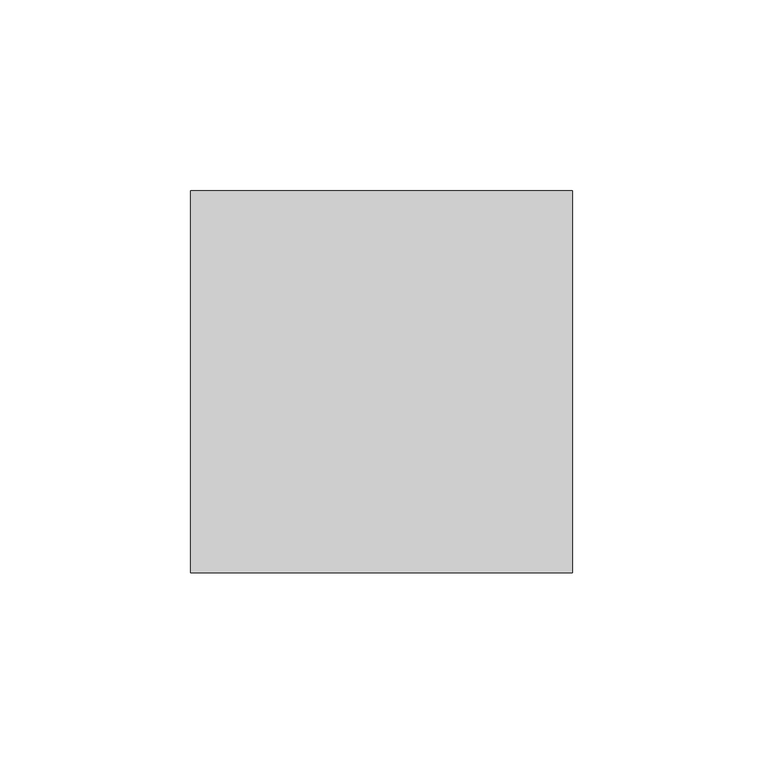
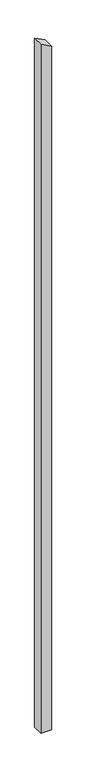
"""IFC4 building model written with IfcOpenShell, lengths in millimetres: column geometry, Holzstütze 159206 : Holzstütze 159206."""

from ifc_helpers import new_model, si_unit, frame, origin, place, context, project, spatial, polyline, outline, extrude, source, transform, mapped, element, save


def column_acd7d749(model_context):
    return source(origin(), model_context, "Body", "SweptSolid", [
        extrude(outline(polyline([(-500.0, 174197.7593015), (-500.0, 174297.7593015), (6345.7118258, 174297.7593015), (6396.6643707, 174197.7593015), (-500.0, 174197.7593015)])), frame((0.0, 35528.3551606, 0.0), z_axis=(0.0, 1.0, 0.0), x_axis=(0.0, 0.0, 1.0)), (0.0, 0.0, 1.0), 100.0),
    ])


if __name__ == "__main__":
    model = new_model("IFC4")
    model_context = context("Model", 3, world=origin())
    ifc_project = project(units=[si_unit("LENGTHUNIT", "METRE", prefix="MILLI")], contexts=[model_context])
    site = spatial("IfcSite", under=ifc_project)
    building = spatial("IfcBuilding", under=site)
    placement = place(None, origin())
    column_shape = column_acd7d749(model_context)
    element("IfcColumn", 1, ObjectType="Holzstütze 159206 : Holzstütze 159206", at=placement, inside=building, context=model_context, shape_type="MappedRepresentation", body=[
        mapped(column_shape, transform((0.0, 0.0, 0.0), x_axis=(1.0, 0.0, 0.0), y_axis=(0.0, 1.0, 0.0), z_axis=(0.0, 0.0, 1.0))),
    ])
    save(model, "model.ifc")

# Revit data of these elements
# Type "Holzstütze 159206 : Holzstütze 159206"
#   Abrechnungsart = "m"
#   Allright_Bauteil_ID = "0152St 0000143482"
#   Bezeichnung = "Holzstütze"
#   Codetext = "ST-HOLZ\\"
#   Gewerk = "Zimmer- und Holzbauarbeiten"
#   Material = "Holz"
#   Objektname = "Stütze"
#   NameOverride = "Holzstütze"
#   Reference = "Holzstütze"
#   Status = "NEW"
#   ThermalTransmittance = 0.0000 BTU/(h·ft²·°F)
#   Roll = 0.00°
#   Slope = 0.00°
#   2D Interaktion = yes
#   IsExternal = yes
#   LoadBearing = yes
# Element 1 (IfcColumn, "Holzstütze 159206 : Holzstütze 159206")
#   Materials on its faces: "holzschalung"
# Materials
#   "holzschalung": class "Unassigned", colour RGB 128 128 128, transparency 0
